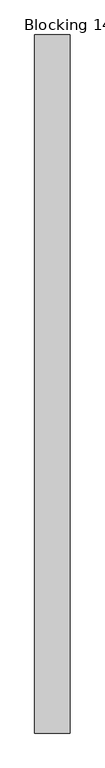
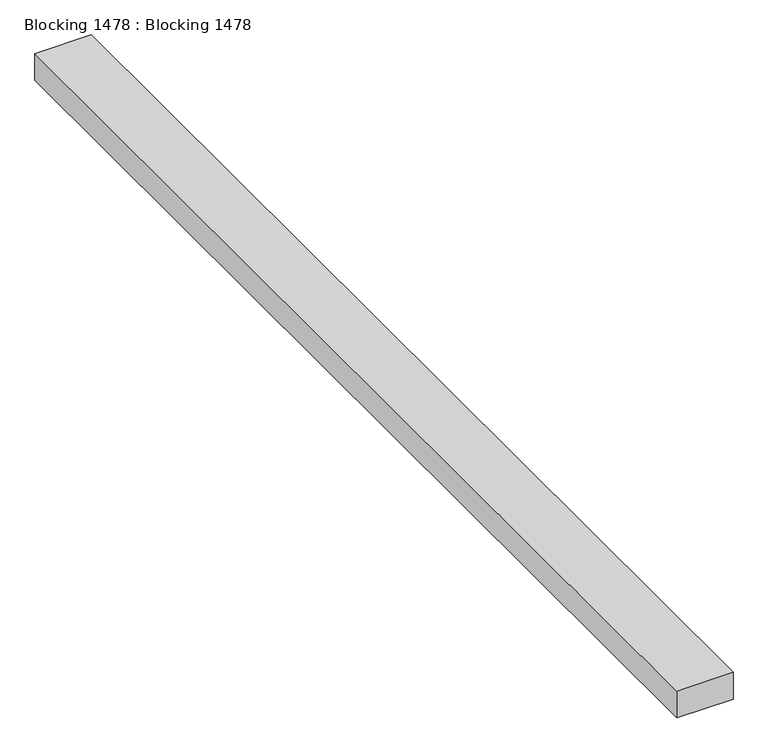
"""IFC4 building model written with IfcOpenShell, lengths in millimetres: proxy geometry, Blocking 1478 : Blocking 1478."""

from ifc_helpers import new_model, si_unit, frame, origin, place, context, project, spatial, polyline, outline, extrude, source, transform, mapped, element, save


def blocking_1478_blocking_1478_60851f08(model_context):
    return source(origin(), model_context, "Body", "SweptSolid", [
        extrude(outline(polyline([(-9787.3237014, 7982.1531721), (-9888.9237014, 7982.1531721), (-9888.9237014, 9982.1531721), (-9787.3237014, 9982.1531721), (-9787.3237014, 7982.1531721)])), frame((0.0, 0.0, 39953.9460083), z_axis=(0.0, 0.0, 1.0), x_axis=(1.0, 0.0, 0.0)), (0.0, 0.0, 1.0), 50.8),
    ])


if __name__ == "__main__":
    model = new_model("IFC4")
    model_context = context("Model", 3, world=origin())
    ifc_project = project(units=[si_unit("LENGTHUNIT", "METRE", prefix="MILLI")], contexts=[model_context])
    site = spatial("IfcSite", under=ifc_project)
    building = spatial("IfcBuilding", under=site)
    placement = place(None, origin())
    blocking_1478_blocking_1478_shape = blocking_1478_blocking_1478_60851f08(model_context)
    element("IfcBuildingElementProxy", 1, Name="Blocking 1478 : Blocking 1478", ObjectType="Blocking 1478 : Blocking 1478", at=placement, inside=building, context=model_context, shape_type="MappedRepresentation", body=[
        mapped(blocking_1478_blocking_1478_shape, transform((0.0, 0.0, 0.0), x_axis=(1.0, 0.0, 0.0), y_axis=(0.0, 1.0, 0.0), z_axis=(0.0, 0.0, 1.0))),
    ])
    save(model, "model.ifc")

# Revit data of these elements
# Type "Blocking 1478 : Blocking 1478"
#   NameOverride = "Blocking"
# Element 1 (IfcBuildingElementProxy, "Blocking 1478 : Blocking 1478")
#   Materials on its faces: "WOOD BLOCKING AS REQUIRED"
# Materials
#   "WOOD BLOCKING AS REQUIRED": class "Unassigned", colour RGB 166 124 85, transparency 0, Cost = 0
